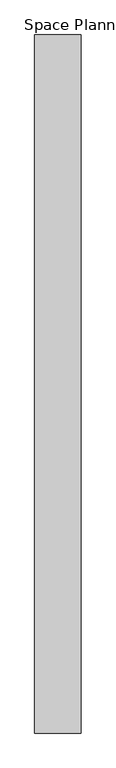
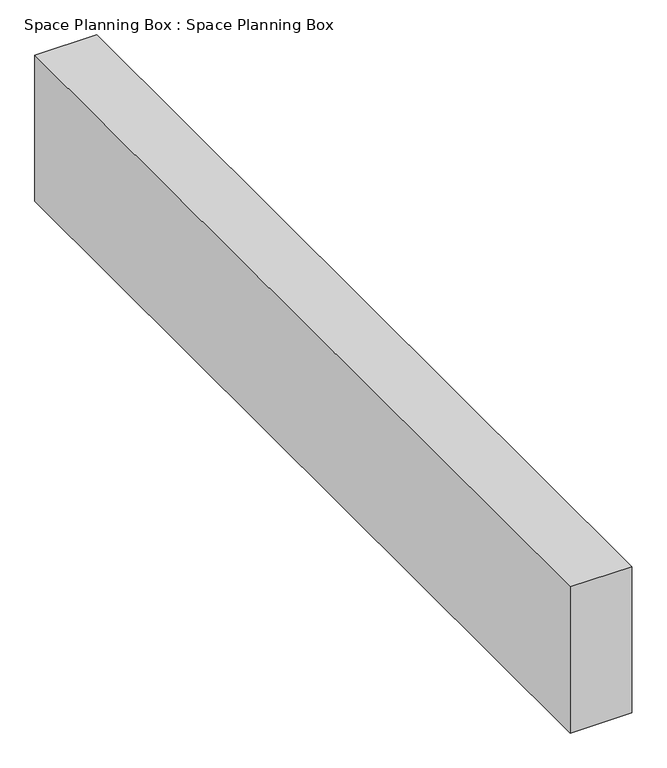
"""IFC4 building model written with IfcOpenShell, lengths in millimetres: proxy geometry, Space Planning Box : Space Planning Box."""

from ifc_helpers import new_model, si_unit, origin, origin_with_axes, place, context, project, spatial, polyline, outline, extrude, source, transform, mapped, element, save


def space_planning_box_space_planning_box_03d31222(model_context):
    return source(origin(), model_context, "Body", "SweptSolid", [
        extrude(outline(polyline([(1200.0, 18000.0), (1200.0, -18000.0), (-1200.0, -18000.0), (-1200.0, 18000.0), (1200.0, 18000.0)])), origin_with_axes(), (0.0, 0.0, 1.0), 6000.0),
    ])


if __name__ == "__main__":
    model = new_model("IFC4")
    model_context = context("Model", 3, world=origin())
    ifc_project = project(units=[si_unit("LENGTHUNIT", "METRE", prefix="MILLI")], contexts=[model_context])
    site = spatial("IfcSite", under=ifc_project)
    building = spatial("IfcBuilding", under=site)
    placement = place(None, origin())
    space_planning_box_space_planning_box_shape = space_planning_box_space_planning_box_03d31222(model_context)
    element("IfcBuildingElementProxy", 1, Name="Space Planning Box : Space Planning Box", ObjectType="Space Planning Box : Space Planning Box", at=placement, inside=building, context=model_context, shape_type="MappedRepresentation", body=[
        mapped(space_planning_box_space_planning_box_shape, transform((0.0, 0.0, 0.0), x_axis=(1.0, 0.0, 0.0), y_axis=(0.0, 1.0, 0.0), z_axis=(0.0, 0.0, 1.0))),
    ])
    save(model, "model.ifc")

# Revit data of these elements
# Type "Space Planning Box : Space Planning Box"
#   Type Comments = "..."
#   Room Name [instance default] = "?"
#   Assembly Code = "..."
#   Width [instance default] = 1524 mm
#   Program Area [instance default] = 0 m²
#   Length [instance default] = 1524 mm
#   Height [instance default] = 1524 mm
#   Area [instance default] = 2.32258 m²
#   Fill Color [instance default] = Cyan
#   Default Elevation = 0
# Element 1 (IfcBuildingElementProxy, "Space Planning Box : Space Planning Box")
#   Room Name = "Corridor"
#   Width = 2400 mm
#   Program Area = 86.4 m²
#   Length = 36000 mm
#   Height = 6000 mm
#   Area = 86.4 m²
#   Fill Color = Lavender
#   Materials on its faces: "Lavender"
# Materials
#   "Cyan": class "Generic", colour RGB 0 255 255, transparency 0.2, Cost = 0
#   "Lavender": class "Generic", colour RGB 186 85 211, transparency 0.2, Cost = 0
